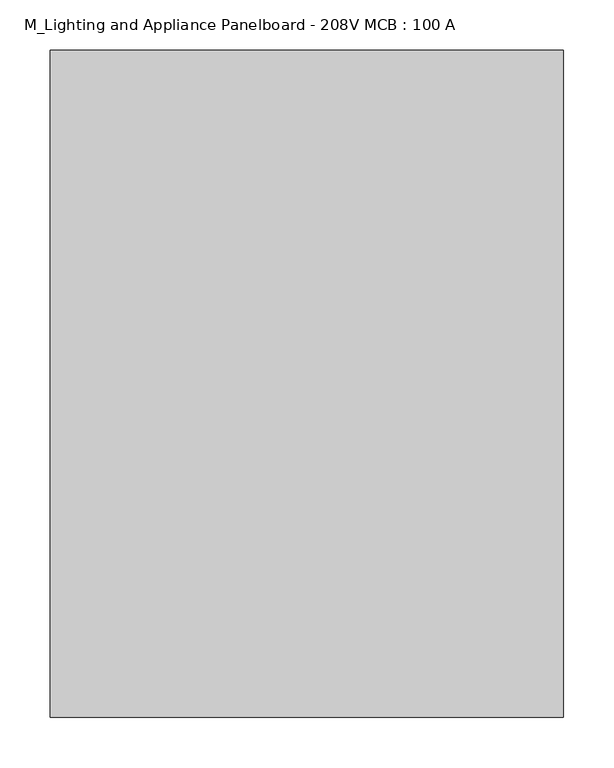
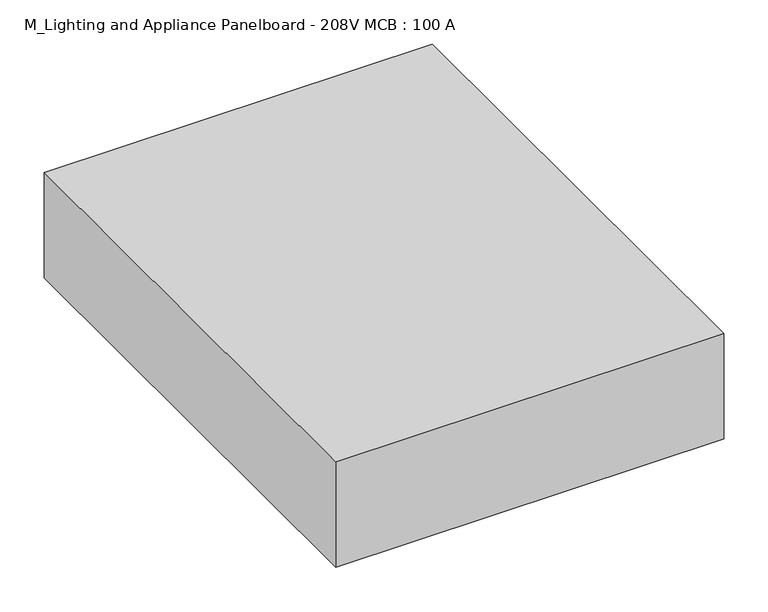
"""IFC4 building model written with IfcOpenShell, lengths in millimetres: proxy geometry, M_Lighting and Appliance Panelboard - 208V MCB : 100 A."""

import ifcopenshell
import ifcopenshell.guid

model = None  # the IFC model being written
_history = None  # IfcOwnerHistory: only IFC2X3 demands one
_inside = {}  # id of a spatial element -> (the spatial element, [elements in it])
_under = {}  # id of a project, library or spatial element -> (it, [spatial elements below it])
_declared = {}  # id of a project -> (the project, [libraries it declares])
_typed = {}  # id of a type object -> (the type object, [elements of that type])
_made_of = {}  # id of a material, layer set ... -> (it, [elements and type objects made of it])


def new_model(schema):
    """Start an empty IFC model of exactly this schema.

    Asked for "IFC4X3", IfcOpenShell would pick the latest addendum, in which some entities
    have other attributes; the version numbers below select the first issue.
    IFC2X3 requires an IfcOwnerHistory on every rooted entity: one is made here for all.
    """
    global model, _history
    if schema == "IFC4X3":
        model = ifcopenshell.file(schema_version=(4, 3, 0, 0))
    else:
        model = ifcopenshell.file(schema=schema)
    _inside.clear()
    _under.clear()
    _declared.clear()
    _typed.clear()
    _made_of.clear()
    _history = None
    if model.schema == "IFC2X3":
        org = make("IfcOrganization", Name="unknown")
        user = make(
            "IfcPersonAndOrganization",
            ThePerson=make("IfcPerson", FamilyName="unknown"),
            TheOrganization=org,
        )
        app = make(
            "IfcApplication",
            ApplicationDeveloper=org,
            Version="unknown",
            ApplicationFullName="unknown",
            ApplicationIdentifier="unknown",
        )
        _history = make(
            "IfcOwnerHistory",
            OwningUser=user,
            OwningApplication=app,
            ChangeAction="ADDED",
            CreationDate=0,
        )
    return model


def make(cls, **values):
    """One entity of the class cls with the attributes given. An attribute that is None is left unset."""
    return model.create_entity(
        cls, **{name: value for name, value in values.items() if value is not None}
    )


def rooted(cls, **values):
    """An entity with a GlobalId (a new one), such as an element, a storey or a relation."""
    return make(cls, GlobalId=ifcopenshell.guid.new(), OwnerHistory=_history, **values)


def si_unit(unit_type, name, prefix=None):
    """IfcSIUnit, for example si_unit("LENGTHUNIT", "METRE", prefix="MILLI")."""
    return make("IfcSIUnit", UnitType=unit_type, Prefix=prefix, Name=name)


def assignment(units):
    """IfcUnitAssignment: the units of a project."""
    return None if units is None else make("IfcUnitAssignment", Units=units)


def point(xyz):
    """IfcCartesianPoint."""
    return None if xyz is None else make("IfcCartesianPoint", Coordinates=xyz)


def direction(xyz):
    """IfcDirection."""
    return None if xyz is None else make("IfcDirection", DirectionRatios=xyz)


def frame(location, z_axis=None, x_axis=None):
    """IfcAxis2Placement3D, a coordinate frame: its origin and axes. An axis left out is left unset."""
    return make(
        "IfcAxis2Placement3D",
        Location=point(location),
        Axis=direction(z_axis),
        RefDirection=direction(x_axis),
    )


def origin():
    """The frame at (0, 0, 0) with its axes left unset."""
    return frame((0.0, 0.0, 0.0))


def place(relative_to, where):
    """IfcLocalPlacement: puts the frame where relative to a parent placement (None: the world)."""
    return make(
        "IfcLocalPlacement", PlacementRelTo=relative_to, RelativePlacement=where
    )


def context(
    kind, dimensions, precision=None, world=None, true_north=None, identifier=None
):
    """IfcGeometricRepresentationContext, for example the 3D "Model" context."""
    return make(
        "IfcGeometricRepresentationContext",
        ContextIdentifier=identifier,
        ContextType=kind,
        CoordinateSpaceDimension=dimensions,
        Precision=precision,
        WorldCoordinateSystem=world,
        TrueNorth=true_north,
    )


def project(units=None, contexts=None):
    """IfcProject with its units and contexts."""
    return rooted(
        "IfcProject",
        Name="project",
        RepresentationContexts=contexts,
        UnitsInContext=assignment(units),
    )


def spatial(cls, under=None, at=None, **own):
    """A site, building, storey or space (cls), placed at a placement, below another one or the project."""
    s = rooted(cls, ObjectPlacement=at, **own)
    if under is not None:
        _under.setdefault(under.id(), (under, []))[1].append(s)
    return s


def polyline(points):
    """IfcPolyline through the points."""
    return make("IfcPolyline", Points=[point(p) for p in points])


def outline(outer, holes=None, kind="AREA"):
    """IfcArbitraryClosedProfileDef: a profile drawn as a closed curve; with holes, ...WithVoids."""
    if holes is None:
        return make("IfcArbitraryClosedProfileDef", ProfileType=kind, OuterCurve=outer)
    return make(
        "IfcArbitraryProfileDefWithVoids",
        ProfileType=kind,
        OuterCurve=outer,
        InnerCurves=holes,
    )


def extrude(swept, where, along, depth):
    """IfcExtrudedAreaSolid: the profile swept, set in the frame where, extruded along a direction by depth."""
    return make(
        "IfcExtrudedAreaSolid",
        SweptArea=swept,
        Position=where,
        ExtrudedDirection=direction(along),
        Depth=depth,
    )


def shape(context_of_items, identifier, shape_type, items):
    """IfcShapeRepresentation: the items that make up one representation, for example the "Body"."""
    return make(
        "IfcShapeRepresentation",
        ContextOfItems=context_of_items,
        RepresentationIdentifier=identifier,
        RepresentationType=shape_type,
        Items=items,
    )


def source(mapping_origin, context_of_items, identifier, shape_type, items):
    """IfcRepresentationMap: a shape defined once, which mapped items show again and again."""
    return make(
        "IfcRepresentationMap",
        MappingOrigin=mapping_origin,
        MappedRepresentation=shape(context_of_items, identifier, shape_type, items),
    )


def transform(
    local_origin,
    x_axis=None,
    y_axis=None,
    z_axis=None,
    scale=None,
    scale2=None,
    scale3=None,
    uniform=True,
):
    """IfcCartesianTransformationOperator3D, or its non-uniform kind. x_axis, y_axis, z_axis: its Axis1, 2, 3."""
    if uniform:
        return make(
            "IfcCartesianTransformationOperator3D",
            Axis1=direction(x_axis),
            Axis2=direction(y_axis),
            LocalOrigin=point(local_origin),
            Scale=scale,
            Axis3=direction(z_axis),
        )
    return make(
        "IfcCartesianTransformationOperator3DnonUniform",
        Axis1=direction(x_axis),
        Axis2=direction(y_axis),
        LocalOrigin=point(local_origin),
        Scale=scale,
        Axis3=direction(z_axis),
        Scale2=scale2,
        Scale3=scale3,
    )


def mapped(mapping_source, mapping_target):
    """IfcMappedItem: shows the shape of a source again, moved by a transform."""
    return make(
        "IfcMappedItem", MappingSource=mapping_source, MappingTarget=mapping_target
    )


def made_of(thing, what):
    """Note that an element or type object is made of a material, layer set ...; save() writes the relation."""
    if what is not None:
        _made_of.setdefault(what.id(), (what, []))[1].append(thing)
    return thing


def element(
    cls,
    number,
    at=None,
    inside=None,
    cuts=None,
    type_object=None,
    material=None,
    context=None,
    identifier="Body",
    shape_type=None,
    held_by="IfcProductDefinitionShape",
    body=None,
    shapes=None,
    **own,
):
    """One element of the class cls, such as IfcWall. Its Tag is "e" and its number.

    at: its placement. inside: the storey or other place that contains it. cuts: it is an
    opening in that element (IfcRelVoidsElement). A single representation is given by context,
    identifier, shape_type and body (its items); several are given by shapes. held_by: the class
    of the entity that holds the representations. save() writes the other relations.
    """
    e = rooted(cls, Tag="e%d" % number, ObjectPlacement=at, **own)
    if body is not None:
        shapes = [shape(context, identifier, shape_type, body)]
    if shapes is not None:
        e.Representation = make(held_by, Representations=shapes)
    if inside is not None:
        _inside.setdefault(inside.id(), (inside, []))[1].append(e)
    if cuts is not None:
        rooted(
            "IfcRelVoidsElement", RelatingBuildingElement=cuts, RelatedOpeningElement=e
        )
    if type_object is not None:
        _typed.setdefault(type_object.id(), (type_object, []))[1].append(e)
    return made_of(e, material)


def aggregate(whole, parts):
    """IfcRelAggregates: a whole, such as a stair, and the parts it consists of."""
    return rooted("IfcRelAggregates", RelatingObject=whole, RelatedObjects=parts)


def save(model, path):
    """Write the relations noted so far, then the file.

    IfcRelAggregates (storeys below a building ...), IfcRelContainedInSpatialStructure (elements
    in a storey), IfcRelDefinesByType, IfcRelAssociatesMaterial and IfcRelDeclares: one each for
    every whole, place, type object, material and project.
    """
    for whole, parts in _under.values():
        aggregate(whole, parts)
    for where, things in _inside.values():
        rooted(
            "IfcRelContainedInSpatialStructure",
            RelatedElements=things,
            RelatingStructure=where,
        )
    for kind, things in _typed.values():
        rooted("IfcRelDefinesByType", RelatedObjects=things, RelatingType=kind)
    for what, things in _made_of.values():
        rooted("IfcRelAssociatesMaterial", RelatedObjects=things, RelatingMaterial=what)
    for by, libraries in _declared.values():
        rooted("IfcRelDeclares", RelatingContext=by, RelatedDefinitions=libraries)
    model.write(path)


def m_lighting_and_appliance_panelboard_208v_mcb_100_a_975063b2(model_context):
    return source(origin(), model_context, "Body", "SweptSolid", [
        extrude(outline(polyline([(349.2594706, 94.0943297), (349.2594706, -566.3056703), (-158.7405294, -566.3056703), (-158.7405294, 94.0943297), (349.2594706, 94.0943297)])), frame((0.0, 0.0, -146.1), z_axis=(0.0, 0.0, 1.0), x_axis=(1.0, 0.0, 0.0)), (0.0, 0.0, 1.0), 146.1),
    ])


if __name__ == "__main__":
    model = new_model("IFC4")
    model_context = context("Model", 3, world=origin())
    ifc_project = project(units=[si_unit("LENGTHUNIT", "METRE", prefix="MILLI")], contexts=[model_context])
    site = spatial("IfcSite", under=ifc_project)
    building = spatial("IfcBuilding", under=site)
    placement = place(None, origin())
    m_lighting_and_appliance_panelboard_208v_mcb_100_a_shape = m_lighting_and_appliance_panelboard_208v_mcb_100_a_975063b2(model_context)
    element("IfcBuildingElementProxy", 1, Name="M_Lighting and Appliance Panelboard - 208V MCB : 100 A", ObjectType="M_Lighting and Appliance Panelboard - 208V MCB : 100 A", at=placement, inside=building, context=model_context, shape_type="MappedRepresentation", body=[
        mapped(m_lighting_and_appliance_panelboard_208v_mcb_100_a_shape, transform((0.0, 0.0, 0.0), x_axis=(1.0, 0.0, 0.0), y_axis=(0.0, 1.0, 0.0), z_axis=(0.0, 0.0, 1.0))),
    ])
    save(model, "model.ifc")

# Revit data of these elements
# Type "M_Lighting and Appliance Panelboard - 208V MCB : 100 A"
#   built-in parameter 1140081 [instance default] = "Recessed"
#   built-in parameter 1140083 [instance default] = "Type 1"
#   Width = 508 mm
#   built-in parameter 1140082 [instance default] = 100 (stored number, unit not read)
#   built-in parameter 1140140 = 100 (stored number, unit not read)
#   Height [instance default] = 584.2 mm
#   Depth = 146.1 mm
#   Default Elevation = 1200 mm
#   42 Circuit Height = 1270 mm
#   30 Circuit Height = 736.6 mm
#   24 Circuit Height = 660.4 mm
#   12 Circuit Height = 584.2 mm
#   built-in parameter 1140079 [instance default] = 12
#   Load Classification = Other
# Element 1 (IfcBuildingElementProxy, "M_Lighting and Appliance Panelboard - 208V MCB : 100 A")
#   Height = 660.4 mm
#   built-in parameter 1140079 = 20
